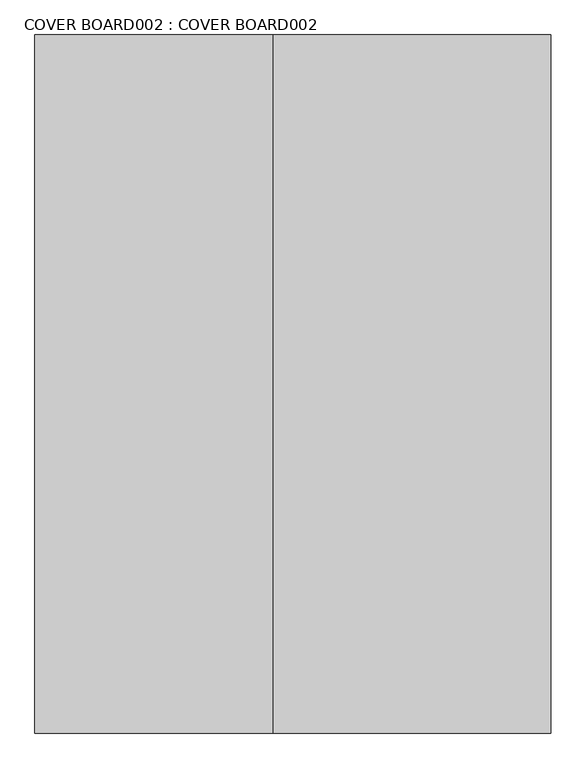
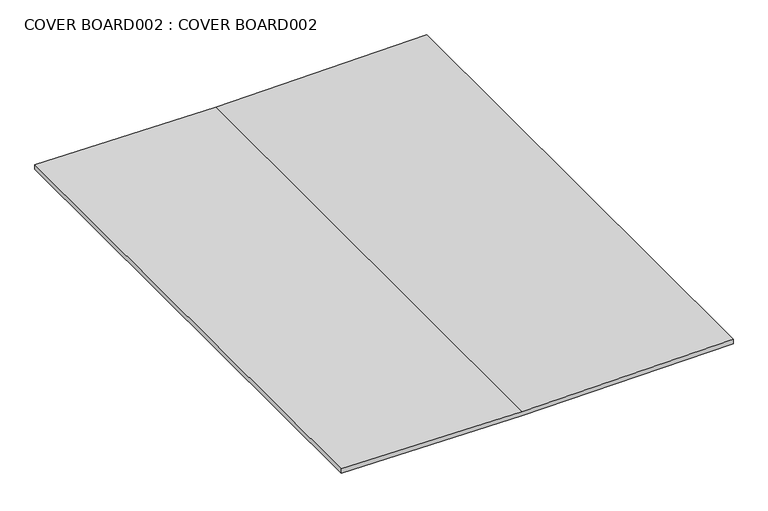
"""IFC4 building model written with IfcOpenShell, lengths in millimetres: proxy geometry, COVER BOARD002 : COVER BOARD002."""

from ifc_helpers import new_model, si_unit, frame, origin, place, context, project, spatial, polyline, outline, extrude, source, transform, mapped, element, save


def cover_board002_cover_board002_e83da0d9(model_context):
    return source(origin(), model_context, "Body", "SweptSolid", [
        extrude(outline(polyline([(40228.1021556, -1886.5629484), (40237.9000089, -2567.3737014), (40220.5682898, -2567.3737014), (40210.7704365, -1886.5629484), (40220.5682898, -1090.0815411), (40237.9000089, -1090.0815411), (40228.1021556, -1886.5629484)])), frame((0.0, 1000.0, 0.0), z_axis=(0.0, 1.0, 0.0), x_axis=(0.0, 0.0, 1.0)), (0.0, 0.0, 1.0), 2000.0),
    ])


if __name__ == "__main__":
    model = new_model("IFC4")
    model_context = context("Model", 3, world=origin())
    ifc_project = project(units=[si_unit("LENGTHUNIT", "METRE", prefix="MILLI")], contexts=[model_context])
    site = spatial("IfcSite", under=ifc_project)
    building = spatial("IfcBuilding", under=site)
    placement = place(None, origin())
    cover_board002_cover_board002_shape = cover_board002_cover_board002_e83da0d9(model_context)
    element("IfcBuildingElementProxy", 1, Name="COVER BOARD002 : COVER BOARD002", ObjectType="COVER BOARD002 : COVER BOARD002", at=placement, inside=building, context=model_context, shape_type="MappedRepresentation", body=[
        mapped(cover_board002_cover_board002_shape, transform((0.0, 0.0, 0.0), x_axis=(1.0, 0.0, 0.0), y_axis=(0.0, 1.0, 0.0), z_axis=(0.0, 0.0, 1.0))),
    ])
    save(model, "model.ifc")

# Revit data of these elements
# Type "COVER BOARD002 : COVER BOARD002"
#   NameOverride = "COVER BOARD002"
# Element 1 (IfcBuildingElementProxy, "COVER BOARD002 : COVER BOARD002")
#   Materials on its faces: "CDX PLYWOOD - SEE STRUCTURAL DWGS"
# Materials
#   "CDX PLYWOOD - SEE STRUCTURAL DWGS": class "Unassigned", colour RGB 202 163 108, transparency 0, Cost = 0
